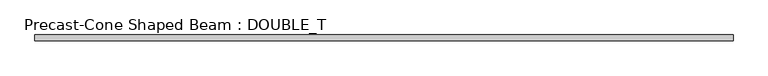
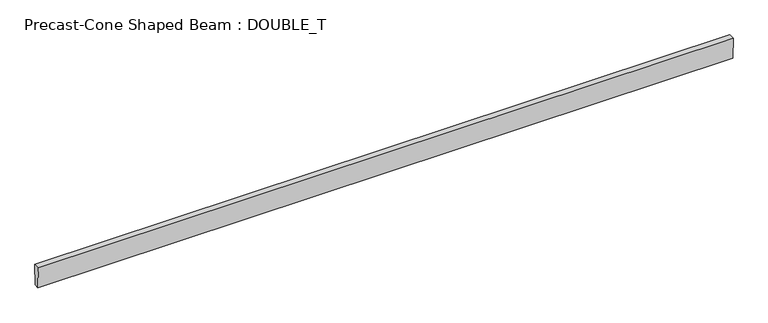
"""IFC4 building model written with IfcOpenShell, lengths in millimetres: beam geometry, Precast-Cone Shaped Beam : DOUBLE_T."""

from ifc_helpers import new_model, si_unit, frame, origin, place, context, project, spatial, polyline, outline, extrude, source, transform, mapped, element, save


def precast_cone_shaped_beam_double_t_c0c18137(model_context):
    return source(origin(), model_context, "Body", "SweptSolid", [
        extrude(outline(polyline([(50.8, -228.6), (-50.8, -228.6), (-63.5, 228.6), (63.5, 228.6), (50.8, -228.6)])), frame((-7378.7, 0.0, 0.0), z_axis=(1.0, 0.0, 0.0), x_axis=(0.0, 1.0, 0.0)), (0.0, 0.0, 1.0), 14909.8),
    ])


if __name__ == "__main__":
    model = new_model("IFC4")
    model_context = context("Model", 3, world=origin())
    ifc_project = project(units=[si_unit("LENGTHUNIT", "METRE", prefix="MILLI")], contexts=[model_context])
    site = spatial("IfcSite", under=ifc_project)
    building = spatial("IfcBuilding", under=site)
    placement = place(None, origin())
    precast_cone_shaped_beam_double_t_shape = precast_cone_shaped_beam_double_t_c0c18137(model_context)
    element("IfcBeam", 1, ObjectType="Precast-Cone Shaped Beam : DOUBLE_T", at=placement, inside=building, context=model_context, shape_type="MappedRepresentation", body=[
        mapped(precast_cone_shaped_beam_double_t_shape, transform((0.0, 0.0, 0.0), x_axis=(1.0, 0.0, 0.0), y_axis=(0.0, 1.0, 0.0), z_axis=(0.0, 0.0, 1.0))),
    ])
    save(model, "model.ifc")

# Revit data of these elements
# Type "Precast-Cone Shaped Beam : DOUBLE_T"
#   Top Width = 0' - 5"
#   Tie Rod Weight [instance default] = 30
#   Tie Rod W [instance default] = 0.0660938 kip
#   Single Rebar Weight [instance default] = 50
#   Single Rebar W [instance default] = 0.110156 kip
#   Rebar Grids Weight [instance default] = 100
#   Rebar Grids W [instance default] = 0.220313 kip
#   Depth = 1' - 6"
#   Bottom Width = 0' - 4"
#   Length [instance default] = 5' - 0"
#   Structural Material [instance default] = Concrete, Precast
#   Assembly Code = ""
# Element 1 (IfcBeam, "Precast-Cone Shaped Beam : DOUBLE_T")
#   Length = 49' - 5"
#   Structural Material = Concrete - Precast Concrete - Normal Weight Concrete - 5 ksi
#   Materials on its faces: "Concrete - Precast Concrete - Normal Weight Concrete - 5 ksi"
# Materials
#   "Concrete, Precast": class "Concrete", colour RGB 198 187 187, transparency 0, Description = "Precast concrete", Cost = 0
#   "Concrete - Precast Concrete - Normal Weight Concrete - 5 ksi": class "Concrete", colour RGB 198 187 187, transparency 0, Cost = 0
